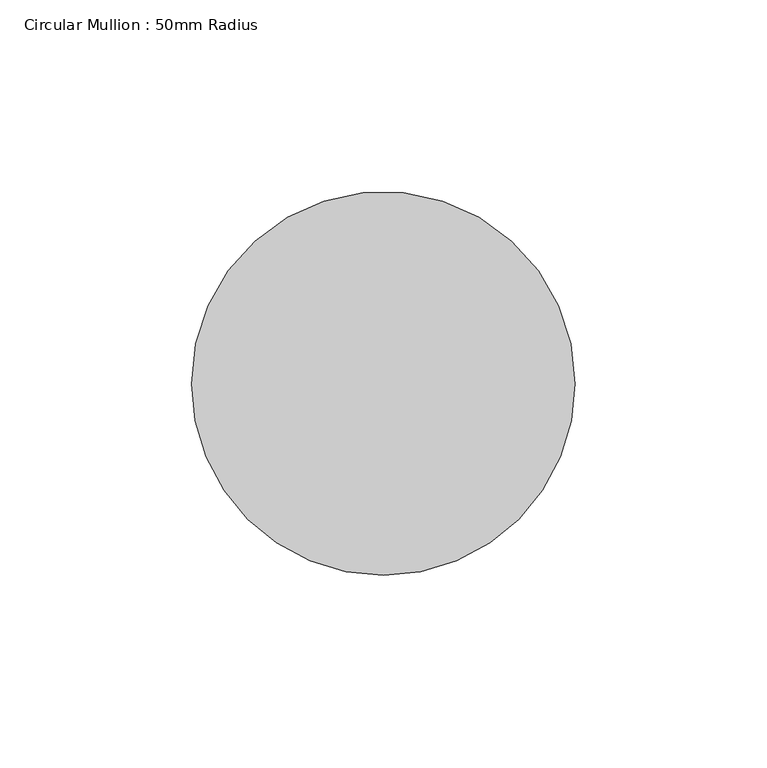
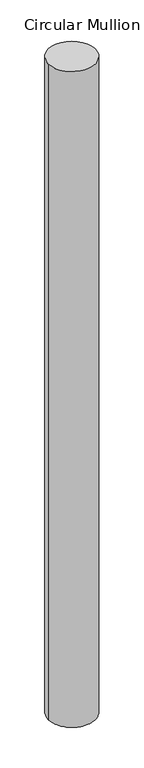
"""IFC4 building model written with IfcOpenShell, lengths in millimetres: member geometry, Circular Mullion : 50mm Radius."""

from ifc_helpers import new_model, si_unit, frame, origin, place, context, project, spatial, ellipse_curve, source, transform, mapped, element, save
from ifc_brep_helpers import plane_surface, cylinder_surface, advanced_brep


def circular_mullion_50mm_radius_c8f20a83(model_context):
    return source(origin(), model_context, "Body", "AdvancedBrep", [
        advanced_brep(
        [(-100.0, 0.0, 0.6042747), (0.0, 0.0, 0.0), (0.0, 0.0, -1478.3651407), (-100.0, 0.0, -1478.6835397)],
        [
            (0, 1, ellipse_curve(frame((-50.0, 0.0, 0.3021374), z_axis=(-0.006042020030486665, -0.014291160384690794, -0.9998796211188676), x_axis=(-0.38936131410647706, -0.920954409189775, 0.015515903814786057)), 50.0060197, 50.0)),
            (1, 2),
            (2, 3, ellipse_curve(frame((-50.0, 0.0, -1478.5243402), z_axis=(-0.0031838836924925518, -0.007530824503408304, 0.9999665742248245), x_axis=(0.38939517435770044, 0.9210344986773663, 0.008176211412910651)), 50.0016713, 50.0)),
            (3, 0),
            (1, 0, ellipse_curve(frame((-50.0, 0.0, 0.3021374), z_axis=(-0.006042020030486665, -0.014291160384690794, -0.9998796211188676), x_axis=(-0.38936131410647706, -0.920954409189775, 0.015515903814786057)), 50.0060197, 50.0)),
            (3, 2, ellipse_curve(frame((-50.0, 0.0, -1478.5243402), z_axis=(-0.0031838836924925518, -0.007530824503408304, 0.9999665742248245), x_axis=(0.38939517435770044, 0.9210344986773663, 0.008176211412910651)), 50.0016713, 50.0)),
        ],
        [
            cylinder_surface(frame((-50.0, 0.0, 0.0), z_axis=(0.0, 0.0, 1.0), x_axis=(1.0, 0.0, 0.0)), 50.0),
            plane_surface(frame((-280.7406992, 118.6916165, 0.0), z_axis=(0.006042020030486665, 0.014291160384690794, 0.9998796211188676), x_axis=(0.3893613141064787, 0.9209544091897743, -0.015515903814788153))),
            plane_surface(frame((-280.7406992, 118.6916165, -1478.3651407), z_axis=(0.0031838836924925526, 0.007530824503408306, -0.9999665742248247), x_axis=(0.3893951743577005, 0.9210344986773664, 0.008176211412901147))),
        ],
        [
            (0, [[1, 2, 3, 4]]),
            (0, [[5, -4, 6, -2]]),
            (1, [[-1, -5]]),
            (2, [[-6, -3]]),
        ],
    ),
    ])


if __name__ == "__main__":
    model = new_model("IFC4")
    model_context = context("Model", 3, world=origin())
    ifc_project = project(units=[si_unit("LENGTHUNIT", "METRE", prefix="MILLI")], contexts=[model_context])
    site = spatial("IfcSite", under=ifc_project)
    building = spatial("IfcBuilding", under=site)
    placement = place(None, origin())
    circular_mullion_50mm_radius_shape = circular_mullion_50mm_radius_c8f20a83(model_context)
    element("IfcMember", 1, ObjectType="Circular Mullion : 50mm Radius", at=placement, inside=building, context=model_context, shape_type="MappedRepresentation", body=[
        mapped(circular_mullion_50mm_radius_shape, transform((0.0, 0.0, 0.0), x_axis=(1.0, 0.0, 0.0), y_axis=(0.0, 1.0, 0.0), z_axis=(0.0, 0.0, 1.0))),
    ])
    save(model, "model.ifc")

# Revit data of these elements
# Type "Circular Mullion : 50mm Radius"
#   built-in parameter 1007350 = 0.164042 (stored number, unit not read)
# Element 1 (IfcMember, "Circular Mullion : 50mm Radius")
#   Materials on its faces: "Aluminium"
# Materials
#   "Aluminium": class "Metal", colour RGB 247 247 247, transparency 0, Description = "Aluminium 6061", Cost = 0
